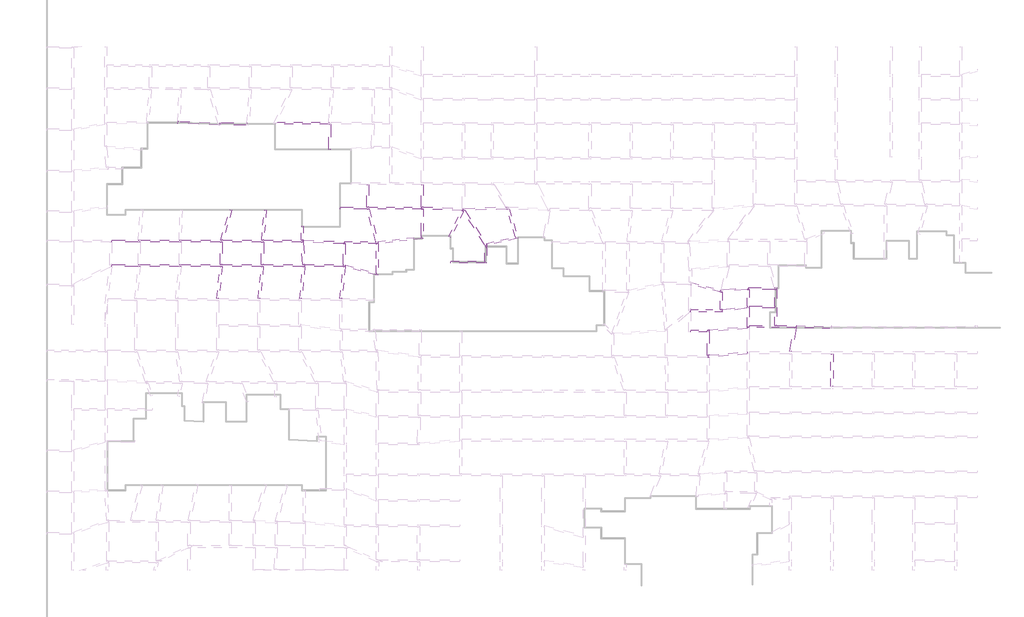
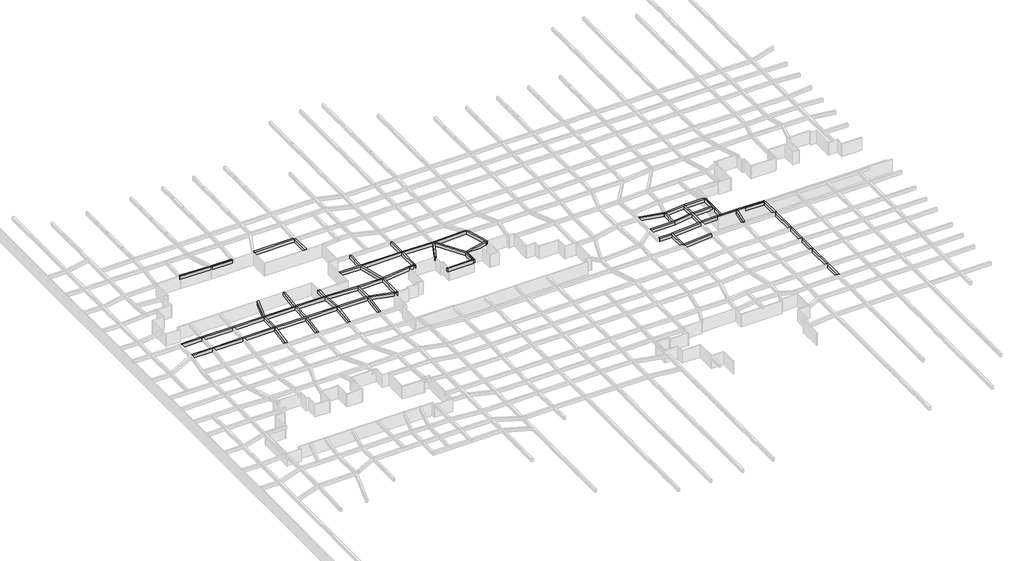
# One storey, part 30 of 45: 53 beams.
# Revit data of these elements (continued)
# Elements 1, 2, 3, 4, 5, 6, 7, 8, 9, 10, 11, 12, 13, 14, 15, 16, 17, 18, 19, 20, 21, 22, 23, 24, 25, 26, 27, 28, 29, 30, 31, 32, 33, 34, 35, 36, 37, 38, 39, 40, 41, 42, 43, 44, 45, 46, 47, 48, 49, 50, 51, 52, 53 (IfcBeam, "混凝土 - 矩形梁 : KL_beam")
#   Comments = ""
#   Structural Material = none
#   Phase Created = 新构造
# Materials
#   "混凝土 - 现场浇注混凝土": class "混凝土", colour RGB 192 192 192, transparency 0
